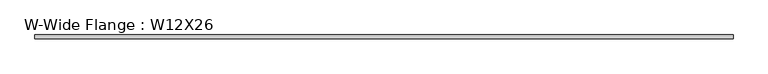
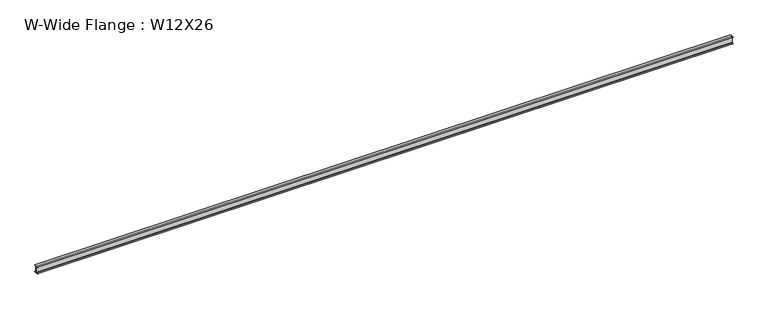
"""IFC4 building model written with IfcOpenShell, lengths in millimetres: beam geometry, W-Wide Flange : W12X26."""

from ifc_helpers import new_model, si_unit, point, frame, frame_2d, origin, place, context, project, spatial, polyline, circle_curve, trimmed, segment, composite_curve, outline, extrude, source, transform, mapped, element, save


def w_wide_flange_w12x26_bec7b074(model_context):
    return source(origin(), model_context, "Body", "SweptSolid", [
        extrude(outline(composite_curve([segment(polyline([(82.4011719, -145.5539063), (82.4011719, -155.178125), (-82.4011719, -155.178125), (-82.4011719, -145.5539063), (-20.2902344, -145.5539063)]), True, "CONTINUOUS"), segment(trimmed(circle_curve(frame_2d((-20.2902344, -128.190625)), 17.3632812), [point((-20.2902344, -145.5539063))], [point((-2.9269531, -128.190625))], True, "CARTESIAN"), True, "CONTINUOUS"), segment(polyline([(-2.9269531, -128.190625), (-2.9269531, 128.190625)]), True, "CONTINUOUS"), segment(trimmed(circle_curve(frame_2d((-20.2902344, 128.190625)), 17.3632812), [point((-2.9269531, 128.190625))], [point((-20.2902344, 145.5539062))], True, "CARTESIAN"), True, "CONTINUOUS"), segment(polyline([(-20.2902344, 145.5539062), (-82.4011719, 145.5539062), (-82.4011719, 155.178125), (82.4011719, 155.178125), (82.4011719, 145.5539062), (20.2902344, 145.5539062)]), True, "CONTINUOUS"), segment(trimmed(circle_curve(frame_2d((20.2902344, 128.190625)), 17.3632812), [point((20.2902344, 145.5539062))], [point((2.9269531, 128.190625))], True, "CARTESIAN"), True, "CONTINUOUS"), segment(polyline([(2.9269531, 128.190625), (2.9269531, -128.190625)]), True, "CONTINUOUS"), segment(trimmed(circle_curve(frame_2d((20.2902344, -128.190625)), 17.3632812), [point((2.9269531, -128.190625))], [point((20.2902344, -145.5539063))], True, "CARTESIAN"), True, "CONTINUOUS"), segment(polyline([(20.2902344, -145.5539063), (82.4011719, -145.5539063)]), True, "CONTINUOUS")], self_intersect=False)), frame((-15000.2301371, 0.0, 0.0), z_axis=(1.0, 0.0, 0.0), x_axis=(0.0, 1.0, 0.0)), (0.0, 0.0, 1.0), 30000.4602742),
    ])


if __name__ == "__main__":
    model = new_model("IFC4")
    model_context = context("Model", 3, world=origin())
    ifc_project = project(units=[si_unit("LENGTHUNIT", "METRE", prefix="MILLI")], contexts=[model_context])
    site = spatial("IfcSite", under=ifc_project)
    building = spatial("IfcBuilding", under=site)
    placement = place(None, origin())
    w_wide_flange_w12x26_shape = w_wide_flange_w12x26_bec7b074(model_context)
    element("IfcBeam", 1, ObjectType="W-Wide Flange : W12X26", at=placement, inside=building, context=model_context, shape_type="MappedRepresentation", body=[
        mapped(w_wide_flange_w12x26_shape, transform((0.0, 0.0, 0.0), x_axis=(1.0, 0.0, 0.0), y_axis=(0.0, 1.0, 0.0), z_axis=(0.0, 0.0, 1.0))),
    ])
    save(model, "model.ifc")

# Revit data of these elements
# Type "W-Wide Flange : W12X26"
#   Assembly Code = "B10"
#   W = 26
#   Length [instance default] = 5' - 0"
#   bf = 0' - 6 125/256"
#   d = 1' - 0 7/32"
#   k = 0' - 1 1/16"
#   k2 = 0' - 0 175/256"
#   tf = 0' - 0 97/256"
#   tw = 0' - 0 59/256"
#   A = 0.053125 SF
#   Structural Material [instance default] = none
